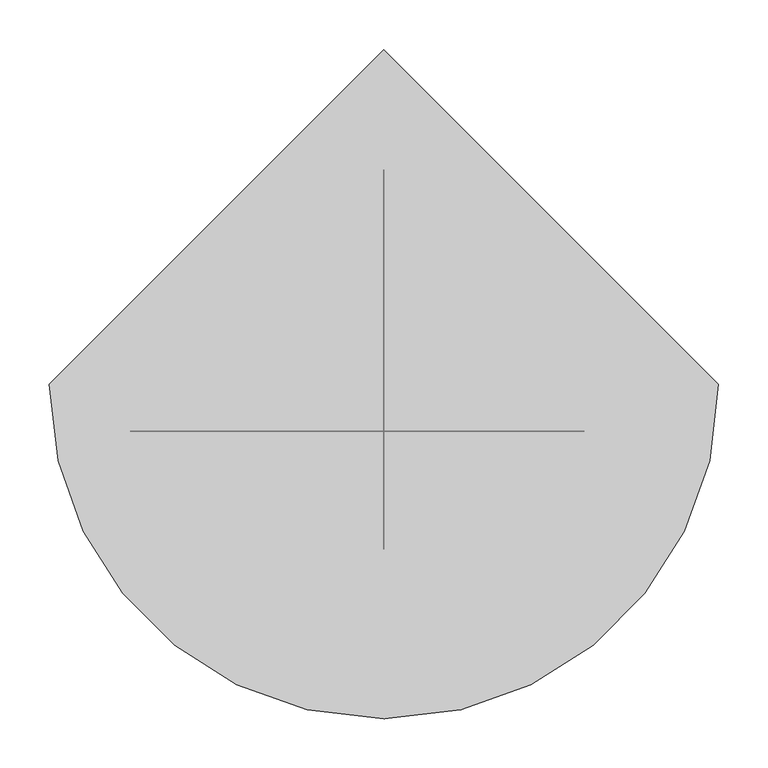
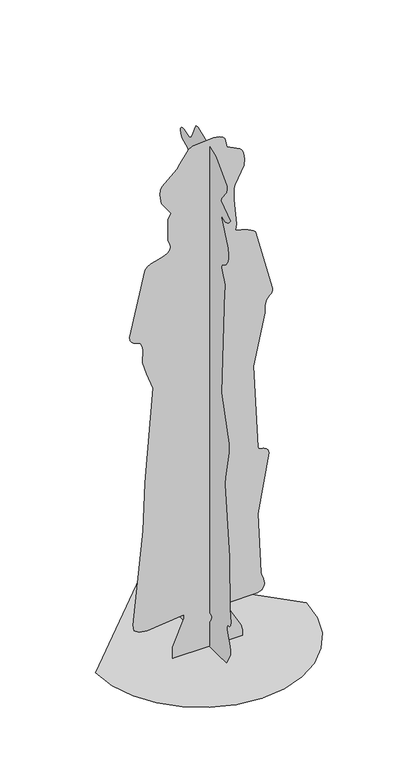
"""IFC4 building model written with IfcOpenShell, lengths in millimetres: proxy geometry, tina 23824 : tina 23824."""

import ifcopenshell
import ifcopenshell.guid

model = None  # the IFC model being written
_history = None  # IfcOwnerHistory: only IFC2X3 demands one
_inside = {}  # id of a spatial element -> (the spatial element, [elements in it])
_under = {}  # id of a project, library or spatial element -> (it, [spatial elements below it])
_declared = {}  # id of a project -> (the project, [libraries it declares])
_typed = {}  # id of a type object -> (the type object, [elements of that type])
_made_of = {}  # id of a material, layer set ... -> (it, [elements and type objects made of it])


def new_model(schema):
    """Start an empty IFC model of exactly this schema.

    Asked for "IFC4X3", IfcOpenShell would pick the latest addendum, in which some entities
    have other attributes; the version numbers below select the first issue.
    IFC2X3 requires an IfcOwnerHistory on every rooted entity: one is made here for all.
    """
    global model, _history
    if schema == "IFC4X3":
        model = ifcopenshell.file(schema_version=(4, 3, 0, 0))
    else:
        model = ifcopenshell.file(schema=schema)
    _inside.clear()
    _under.clear()
    _declared.clear()
    _typed.clear()
    _made_of.clear()
    _history = None
    if model.schema == "IFC2X3":
        org = make("IfcOrganization", Name="unknown")
        user = make(
            "IfcPersonAndOrganization",
            ThePerson=make("IfcPerson", FamilyName="unknown"),
            TheOrganization=org,
        )
        app = make(
            "IfcApplication",
            ApplicationDeveloper=org,
            Version="unknown",
            ApplicationFullName="unknown",
            ApplicationIdentifier="unknown",
        )
        _history = make(
            "IfcOwnerHistory",
            OwningUser=user,
            OwningApplication=app,
            ChangeAction="ADDED",
            CreationDate=0,
        )
    return model


def make(cls, **values):
    """One entity of the class cls with the attributes given. An attribute that is None is left unset."""
    return model.create_entity(
        cls, **{name: value for name, value in values.items() if value is not None}
    )


def rooted(cls, **values):
    """An entity with a GlobalId (a new one), such as an element, a storey or a relation."""
    return make(cls, GlobalId=ifcopenshell.guid.new(), OwnerHistory=_history, **values)


def si_unit(unit_type, name, prefix=None):
    """IfcSIUnit, for example si_unit("LENGTHUNIT", "METRE", prefix="MILLI")."""
    return make("IfcSIUnit", UnitType=unit_type, Prefix=prefix, Name=name)


def assignment(units):
    """IfcUnitAssignment: the units of a project."""
    return None if units is None else make("IfcUnitAssignment", Units=units)


def point(xyz):
    """IfcCartesianPoint."""
    return None if xyz is None else make("IfcCartesianPoint", Coordinates=xyz)


def direction(xyz):
    """IfcDirection."""
    return None if xyz is None else make("IfcDirection", DirectionRatios=xyz)


def frame(location, z_axis=None, x_axis=None):
    """IfcAxis2Placement3D, a coordinate frame: its origin and axes. An axis left out is left unset."""
    return make(
        "IfcAxis2Placement3D",
        Location=point(location),
        Axis=direction(z_axis),
        RefDirection=direction(x_axis),
    )


def origin():
    """The frame at (0, 0, 0) with its axes left unset."""
    return frame((0.0, 0.0, 0.0))


def place(relative_to, where):
    """IfcLocalPlacement: puts the frame where relative to a parent placement (None: the world)."""
    return make(
        "IfcLocalPlacement", PlacementRelTo=relative_to, RelativePlacement=where
    )


def context(
    kind, dimensions, precision=None, world=None, true_north=None, identifier=None
):
    """IfcGeometricRepresentationContext, for example the 3D "Model" context."""
    return make(
        "IfcGeometricRepresentationContext",
        ContextIdentifier=identifier,
        ContextType=kind,
        CoordinateSpaceDimension=dimensions,
        Precision=precision,
        WorldCoordinateSystem=world,
        TrueNorth=true_north,
    )


def project(units=None, contexts=None):
    """IfcProject with its units and contexts."""
    return rooted(
        "IfcProject",
        Name="project",
        RepresentationContexts=contexts,
        UnitsInContext=assignment(units),
    )


def spatial(cls, under=None, at=None, **own):
    """A site, building, storey or space (cls), placed at a placement, below another one or the project."""
    s = rooted(cls, ObjectPlacement=at, **own)
    if under is not None:
        _under.setdefault(under.id(), (under, []))[1].append(s)
    return s


def point_list(points):
    """IfcCartesianPointList2D or 3D."""
    cls = (
        "IfcCartesianPointList2D" if len(points[0]) == 2 else "IfcCartesianPointList3D"
    )
    return make(cls, CoordList=points)


def triangles(points, corners, closed=None, point_numbers=None):
    """IfcTriangulatedFaceSet: each triangle names its three corners, points numbered from 1."""
    return make(
        "IfcTriangulatedFaceSet",
        Coordinates=point_list(points),
        Closed=closed,
        CoordIndex=corners,
        PnIndex=point_numbers,
    )


def shape(context_of_items, identifier, shape_type, items):
    """IfcShapeRepresentation: the items that make up one representation, for example the "Body"."""
    return make(
        "IfcShapeRepresentation",
        ContextOfItems=context_of_items,
        RepresentationIdentifier=identifier,
        RepresentationType=shape_type,
        Items=items,
    )


def source(mapping_origin, context_of_items, identifier, shape_type, items):
    """IfcRepresentationMap: a shape defined once, which mapped items show again and again."""
    return make(
        "IfcRepresentationMap",
        MappingOrigin=mapping_origin,
        MappedRepresentation=shape(context_of_items, identifier, shape_type, items),
    )


def transform(
    local_origin,
    x_axis=None,
    y_axis=None,
    z_axis=None,
    scale=None,
    scale2=None,
    scale3=None,
    uniform=True,
):
    """IfcCartesianTransformationOperator3D, or its non-uniform kind. x_axis, y_axis, z_axis: its Axis1, 2, 3."""
    if uniform:
        return make(
            "IfcCartesianTransformationOperator3D",
            Axis1=direction(x_axis),
            Axis2=direction(y_axis),
            LocalOrigin=point(local_origin),
            Scale=scale,
            Axis3=direction(z_axis),
        )
    return make(
        "IfcCartesianTransformationOperator3DnonUniform",
        Axis1=direction(x_axis),
        Axis2=direction(y_axis),
        LocalOrigin=point(local_origin),
        Scale=scale,
        Axis3=direction(z_axis),
        Scale2=scale2,
        Scale3=scale3,
    )


def mapped(mapping_source, mapping_target):
    """IfcMappedItem: shows the shape of a source again, moved by a transform."""
    return make(
        "IfcMappedItem", MappingSource=mapping_source, MappingTarget=mapping_target
    )


def made_of(thing, what):
    """Note that an element or type object is made of a material, layer set ...; save() writes the relation."""
    if what is not None:
        _made_of.setdefault(what.id(), (what, []))[1].append(thing)
    return thing


def element(
    cls,
    number,
    at=None,
    inside=None,
    cuts=None,
    type_object=None,
    material=None,
    context=None,
    identifier="Body",
    shape_type=None,
    held_by="IfcProductDefinitionShape",
    body=None,
    shapes=None,
    **own,
):
    """One element of the class cls, such as IfcWall. Its Tag is "e" and its number.

    at: its placement. inside: the storey or other place that contains it. cuts: it is an
    opening in that element (IfcRelVoidsElement). A single representation is given by context,
    identifier, shape_type and body (its items); several are given by shapes. held_by: the class
    of the entity that holds the representations. save() writes the other relations.
    """
    e = rooted(cls, Tag="e%d" % number, ObjectPlacement=at, **own)
    if body is not None:
        shapes = [shape(context, identifier, shape_type, body)]
    if shapes is not None:
        e.Representation = make(held_by, Representations=shapes)
    if inside is not None:
        _inside.setdefault(inside.id(), (inside, []))[1].append(e)
    if cuts is not None:
        rooted(
            "IfcRelVoidsElement", RelatingBuildingElement=cuts, RelatedOpeningElement=e
        )
    if type_object is not None:
        _typed.setdefault(type_object.id(), (type_object, []))[1].append(e)
    return made_of(e, material)


def aggregate(whole, parts):
    """IfcRelAggregates: a whole, such as a stair, and the parts it consists of."""
    return rooted("IfcRelAggregates", RelatingObject=whole, RelatedObjects=parts)


def save(model, path):
    """Write the relations noted so far, then the file.

    IfcRelAggregates (storeys below a building ...), IfcRelContainedInSpatialStructure (elements
    in a storey), IfcRelDefinesByType, IfcRelAssociatesMaterial and IfcRelDeclares: one each for
    every whole, place, type object, material and project.
    """
    for whole, parts in _under.values():
        aggregate(whole, parts)
    for where, things in _inside.values():
        rooted(
            "IfcRelContainedInSpatialStructure",
            RelatedElements=things,
            RelatingStructure=where,
        )
    for kind, things in _typed.values():
        rooted("IfcRelDefinesByType", RelatedObjects=things, RelatingType=kind)
    for what, things in _made_of.values():
        rooted("IfcRelAssociatesMaterial", RelatedObjects=things, RelatingMaterial=what)
    for by, libraries in _declared.values():
        rooted("IfcRelDeclares", RelatingContext=by, RelatedDefinitions=libraries)
    model.write(path)


def entourage_2895b76d(model_context):
    return source(origin(), model_context, "Body", "Tessellation", [
        triangles([(-118.6024808, -47.6347378, 38.0857045), (-82.4820657, -47.6347378, 123.5964438), (-82.4078333, -47.6347378, 135.8076171), (-201.8741786, -47.6347378, 123.6873721), (-226.8996859, -47.6347378, 127.3924875), (-242.8002052, -47.6347378, 138.1060324), (-245.9828961, -47.6347378, 157.9872498), (-214.4620912, -47.6347378, 467.6612801), (-208.2590723, -47.6347378, 628.7997002), (-182.2156765, -47.6347378, 942.5936279), (-202.381742, -47.6347378, 998.3094131), (-215.4855752, -47.6347378, 1039.6297834), (-215.821474, -47.6347378, 1048.3149364), (-215.4215529, -47.6347378, 1056.8906485), (-214.7395452, -47.6347378, 1065.4273367), (-214.2301286, -47.6347378, 1073.9983252), (-214.3442568, -47.6347378, 1082.6741764), (-215.5356812, -47.6347378, 1091.525453), (-218.2581349, -47.6347378, 1100.6244616), (-222.7723761, -47.6347378, 1107.0752306), (-229.4309994, -47.6347378, 1111.2517199), (-237.153911, -47.6347378, 1114.3369967), (-244.8601449, -47.6347378, 1117.5141283), (-251.4686441, -47.6347378, 1121.9680716), (-255.900314, -47.6347378, 1128.8818211), (-257.0722446, -47.6347378, 1139.4385895), (-207.1678598, -47.6347378, 1352.9180008), (-199.4588645, -47.6347378, 1360.8821949), (-187.4852313, -47.6347378, 1366.7168678), (-173.049866, -47.6347378, 1371.2959488), (-157.9566194, -47.6347378, 1375.4901695), (-144.0093421, -47.6347378, 1380.175058), (-133.0118575, -47.6347378, 1386.2222179), (-126.7670806, -47.6347378, 1394.5047066), (-125.4318332, -47.6347378, 1401.2801651), (-127.4128987, -47.6347378, 1413.4282608), (-129.6649143, -47.6347378, 1418.6895676), (-132.0486895, -47.6347378, 1423.3336155), (-134.0325437, -47.6347378, 1427.3050301), (-132.6945168, -47.6347378, 1497.2715443), (-129.1053917, -47.6347378, 1508.7544189), (-123.9945118, -47.6347378, 1516.4930454), (-154.1540899, -47.6347378, 1559.4808285), (-159.7585988, -47.6347378, 1590.521957), (-157.2634749, -47.6347378, 1607.9849899), (-153.0368979, -47.6347378, 1617.2900906), (-104.5874569, -47.6347378, 1660.6611351), (-95.4448464, -47.6347378, 1675.8824444), (-68.2647649, -47.6347378, 1712.8963188), (-54.7860727, -47.6347378, 1720.8057198), (13.793251, -47.6347378, 1725.7013512), (32.0821851, -47.6347378, 1722.1345631), (43.5352696, -47.6347378, 1716.6933254), (49.9127328, -47.6347378, 1709.5716671), (56.2159682, -47.6347378, 1680.0680901), (98.2526783, -47.6347378, 1658.6643093), (104.3554853, -47.6347378, 1651.6019497), (108.8919907, -47.6347378, 1641.2540348), (113.2271458, -47.6347378, 1617.3336926), (111.7879713, -47.6347378, 1597.1945148), (82.8123962, -47.6347378, 1541.3868748), (78.3955873, -47.6347378, 1530.355862), (78.221143, -47.6347378, 1494.4090736), (81.1505245, -47.6347378, 1473.5952278), (87.0705392, -47.6347378, 1407.3950535), (83.9407248, -47.6347378, 1386.1879177), (93.3691283, -47.6347378, 1383.7559441), (103.6669826, -47.6347378, 1380.9944847), (114.2487677, -47.6347378, 1377.7940987), (124.5280548, -47.6347378, 1374.0491238), (133.9211951, -47.6347378, 1369.6499737), (141.84176, -47.6347378, 1364.4908409), (147.707027, -47.6347378, 1358.4631565), (203.1565494, -47.6347378, 1147.7562504), (202.6489859, -47.6347378, 1140.2068565), (200.5667729, -47.6347378, 1134.3935486), (197.3998514, -47.6347378, 1129.8329258), (193.6427769, -47.6347378, 1126.0442762), (189.7864171, -47.6347378, 1122.5442719), (186.3244191, -47.6347378, 1118.8530727), (183.7485589, -47.6347378, 1114.4863335), (180.7412388, -47.6347378, 1104.3026527), (179.3224846, -47.6347378, 1093.7014103), (178.983788, -47.6347378, 1082.7502619), (179.2129891, -47.6347378, 1071.5217321), (142.1618895, -47.6347378, 903.7795), (156.0237977, -47.6347378, 623.7611996), (158.5087296, -47.6347378, 617.7901251), (163.2567864, -47.6347378, 614.8626148), (169.444036, -47.6347378, 613.3956259), (176.2446201, -47.6347378, 611.8079321), (182.8317907, -47.6347378, 608.5166722), (188.3815792, -47.6347378, 601.9378587), (192.0662743, -47.6347378, 590.4912827), (156.0237977, -47.6347378, 396.418899), (165.8020344, -47.6347378, 192.9106632), (168.1922955, -47.6347378, 185.5199261), (170.9797162, -47.6347378, 177.5863805), (173.6307353, -47.6347378, 169.2955712), (175.6127183, -47.6347378, 160.8312623), (176.3903053, -47.6347378, 152.379934), (175.4317882, -47.6347378, 144.1253234), (168.3491173, -47.6347378, 133.8915095), (154.6421597, -47.6347378, 127.7701444), (58.9885369, -47.6347378, 127.4899107), (56.2159682, -47.6347378, 116.4005713), (101.0707112, -47.6347378, 37.0993457), (106.6641016, -47.6347378, 18.0541737), (105.8020812, -47.6347378, 0.0), (-118.3148258, -47.6347378, 0.0), (0.0, -54.5513123, 115.1627471), (0.0, -59.6705447, 112.2277973), (0.0, -61.6061461, 107.3080667), (0.0, -59.5796073, 99.6946324), (0.0, -52.8142817, 88.6758101), (0.0, -44.5346181, 79.7484662), (0.0, -38.0847779, 77.4212917), (0.0, -33.3088703, 80.3915047), (0.0, -30.0537933, 87.3554056), (0.0, -27.8620893, 119.17314), (0.0, -145.2091144, 6.8673968), (0.0, -161.5494597, 35.0431167), (0.0, -163.7123909, 41.543994), (0.0, -165.0513535, 56.4646448), (0.0, -162.6425252, 70.0333433), (0.0, -147.9891046, 107.0380432), (0.0, -145.6442986, 119.6101773), (0.0, -147.0779048, 133.0350483), (0.0, -159.447753, 133.9267635), (0.0, -165.7983101, 141.1708889), (0.0, -167.6643299, 152.8364559), (0.0, -161.6821551, 195.066182), (0.0, -158.8307121, 370.4998052), (0.0, -134.8528152, 604.4088561), (0.0, -137.4657826, 630.1117567), (0.0, -156.469192, 724.2417669), (0.0, -156.1305136, 755.5583874), (0.0, -114.2079362, 903.3962385), (0.0, -130.4434278, 1258.6544231), (0.0, -135.0133342, 1270.3422272), (0.0, -134.2635979, 1282.5153214), (0.0, -115.83826, 1329.7483395), (0.0, -116.8218301, 1339.6090748), (0.0, -129.4932496, 1346.1220493), (0.0, -140.4582598, 1355.1042046), (0.0, -148.9049463, 1366.6277744), (0.0, -154.0176883, 1380.767173), (0.0, -154.9836359, 1397.5927448), (0.0, -150.9899389, 1417.1778866), (0.0, -111.0354464, 1505.4037514), (0.0, -130.1557727, 1498.7358444), (0.0, -138.0614948, 1498.201284), (0.0, -145.1534401, 1499.6340454), (0.0, -151.6478203, 1503.109996), (0.0, -157.7617548, 1508.7042767), (0.0, -163.7123909, 1516.4930454), (0.0, -111.0354464, 1555.307246), (0.0, -115.3928657, 1565.6672241), (0.0, -142.5367576, 1601.7699623), (0.0, -145.4540849, 1612.318301), (0.0, -144.305336, 1624.6185677), (0.0, -83.3116117, 1688.3858963), (0.0, 16.4971557, 1727.1999516), (0.0, 26.1092848, 1726.2803856), (0.0, 33.1455581, 1716.0308659), (0.0, 45.9051286, 1684.0145061), (0.0, 54.8352521, 1670.4856808), (0.0, 67.6013152, 1664.1007507), (0.0, 95.5905225, 1672.8907665), (0.0, 103.6679091, 1673.2759174), (0.0, 109.6602941, 1670.5970112), (0.0, 113.1909561, 1665.3155022), (0.0, 113.8794588, 1657.8950249), (0.0, 111.3472188, 1648.7960163), (0.0, 105.2165701, 1638.4815296), (0.0, 102.2760519, 1635.7719566), (0.0, 74.7192446, 1624.6185677), (0.0, 65.7640681, 1614.5842964), (0.0, 62.4319768, 1602.0937798), (0.0, 63.3793663, 1588.1734085), (0.0, 83.0360199, 1538.6726509), (0.0, 77.4992394, 1529.7277027), (0.0, 75.4829062, 1476.4142418), (0.0, 71.8251217, 1469.4614685), (0.0, 16.4971557, 1466.5886787), (0.0, 16.4971557, 1366.7799454), (0.0, 18.8484578, 1360.1880512), (0.0, 52.539621, 1327.9657448), (0.0, 105.3622552, 1231.39911), (0.0, 120.552925, 982.93041), (0.0, 166.2103126, 823.3777943), (0.0, 167.4165798, 801.2900436), (0.0, 164.7089689, 783.190349), (0.0, 144.2060507, 730.9643944), (0.0, 144.0306798, 718.0239052), (0.0, 171.7554501, 645.9398603), (0.0, 186.7994991, 525.8657578), (0.0, 217.1038267, 449.5254684), (0.0, 217.3831338, 436.7788628), (0.0, 207.796982, 424.1436602), (0.0, 134.1002812, 404.8247449), (0.0, 105.2156435, 404.7365962), (0.0, 152.8058437, 209.5887513), (0.0, 152.0635198, 186.4487575), (0.0, 141.0131496, 169.2779487), (0.0, 115.8067122, 150.5668179), (0.0, 57.3786288, 128.2990456), (0.0, 49.7670522, 127.4899107), (0.0, 46.9944834, 116.4005713), (0.0, 56.6344519, 98.9615921), (0.0, 86.162119, 72.0468878), (0.0, 157.830428, 32.1499203), (0.0, 159.4356897, 29.2929136), (0.0, 159.4867404, 24.5244297), (0.0, 158.6367741, 18.6443187), (0.0, 157.534425, 12.4515065), (0.0, 156.8329416, 6.7467698), (0.0, 157.1827568, 2.3299599), (0.0, 159.2361925, 0.0), (0.0, -142.9329725, 0.0), (-339.3492356, 0.0, 0.0), (-330.3783079, -77.756264, 0.0), (-304.8276146, -149.1629065, 0.0), (-264.7450685, -212.1748216, 0.0), (-212.1748216, -264.7450685, 0.0), (-149.1629065, -304.8276146, 0.0), (-77.756264, -330.3783079, 0.0), (0.0, -339.3492356, 0.0), (77.756264, -330.3783079, 0.0), (149.1629065, -304.8276146, 0.0), (212.1748216, -264.7450685, 0.0), (264.7450685, -212.1748216, 0.0), (304.8276146, -149.1629065, 0.0), (330.3783079, -77.756264, 0.0), (339.3492356, 0.0, 0.0), (0.0, 339.3492356, 0.0)], [[108, 109, 110], [107, 108, 110], [107, 110, 1], [106, 107, 1], [106, 1, 2], [106, 2, 3], [105, 106, 3], [5, 6, 7], [4, 5, 7], [4, 7, 8], [3, 4, 8], [105, 3, 8], [104, 105, 8], [103, 104, 8], [102, 103, 8], [101, 102, 8], [100, 101, 8], [99, 100, 8], [98, 99, 8], [97, 98, 8], [96, 97, 8], [95, 96, 8], [95, 8, 9], [94, 95, 9], [93, 94, 9], [92, 93, 9], [91, 92, 9], [90, 91, 9], [89, 90, 9], [88, 89, 9], [87, 88, 9], [86, 87, 9], [86, 9, 10], [86, 10, 11], [85, 86, 11], [84, 85, 11], [84, 11, 12], [84, 12, 13], [84, 13, 14], [84, 14, 15], [84, 15, 16], [84, 16, 17], [83, 84, 17], [83, 17, 18], [82, 83, 18], [82, 18, 19], [81, 82, 19], [80, 81, 19], [80, 19, 20], [79, 80, 20], [78, 79, 20], [77, 78, 20], [76, 77, 20], [75, 76, 20], [74, 75, 20], [73, 74, 20], [72, 73, 20], [71, 72, 20], [70, 71, 20], [69, 70, 20], [68, 69, 20], [67, 68, 20], [66, 67, 20], [66, 20, 21], [66, 21, 22], [66, 22, 23], [66, 23, 24], [66, 24, 25], [66, 25, 26], [66, 26, 27], [66, 27, 28], [66, 28, 29], [66, 29, 30], [66, 30, 31], [66, 31, 32], [66, 32, 33], [66, 33, 34], [66, 34, 35], [65, 66, 35], [64, 65, 35], [64, 35, 36], [64, 36, 37], [63, 64, 37], [63, 37, 38], [63, 38, 39], [63, 39, 40], [63, 40, 41], [63, 41, 42], [62, 63, 42], [61, 62, 42], [61, 42, 43], [61, 43, 44], [61, 44, 45], [61, 45, 46], [61, 46, 47], [61, 47, 48], [60, 61, 48], [59, 60, 48], [58, 59, 48], [57, 58, 48], [56, 57, 48], [55, 56, 48], [55, 48, 49], [55, 49, 50], [55, 50, 51], [55, 51, 52], [55, 52, 53], [55, 53, 54], [218, 219, 220], [115, 123, 124], [115, 124, 125], [114, 115, 125], [114, 125, 126], [113, 114, 126], [113, 126, 127], [217, 218, 220], [155, 156, 157], [122, 123, 115], [122, 115, 116], [121, 122, 116], [216, 217, 220], [215, 216, 220], [214, 215, 220], [213, 214, 220], [212, 213, 220], [211, 212, 220], [210, 211, 220], [210, 220, 121], [209, 210, 121], [112, 113, 127], [112, 127, 128], [183, 184, 185], [180, 181, 182], [121, 116, 117], [209, 121, 117], [209, 117, 118], [209, 118, 119], [209, 119, 120], [208, 209, 120], [154, 155, 157], [153, 154, 157], [152, 153, 157], [151, 152, 157], [150, 151, 157], [163, 164, 165], [162, 163, 165], [162, 165, 166], [128, 129, 130], [128, 130, 131], [112, 128, 131], [112, 131, 132], [111, 112, 132], [120, 111, 132], [208, 120, 132], [208, 132, 133], [207, 208, 133], [206, 207, 133], [205, 206, 133], [204, 205, 133], [203, 204, 133], [202, 203, 133], [202, 133, 134], [182, 183, 185], [202, 134, 135], [180, 182, 185], [162, 166, 167], [161, 162, 167], [160, 161, 167], [159, 160, 167], [158, 159, 167], [157, 158, 167], [157, 167, 168], [150, 157, 168], [201, 202, 135], [200, 201, 135], [199, 200, 135], [198, 199, 135], [197, 198, 135], [196, 197, 135], [195, 196, 135], [195, 135, 136], [194, 195, 136], [194, 136, 137], [193, 194, 137], [192, 193, 137], [191, 192, 137], [191, 137, 138], [190, 191, 138], [190, 138, 139], [189, 190, 139], [188, 189, 139], [188, 139, 140], [188, 140, 141], [188, 141, 142], [187, 188, 142], [187, 142, 143], [186, 187, 143], [185, 186, 143], [185, 143, 144], [185, 144, 145], [185, 145, 146], [185, 146, 147], [185, 147, 148], [185, 148, 149], [185, 149, 150], [185, 150, 168], [170, 171, 172], [170, 172, 173], [169, 170, 173], [169, 173, 174], [169, 174, 175], [169, 175, 176], [168, 169, 176], [168, 176, 177], [168, 177, 178], [185, 168, 178], [185, 178, 179], [180, 185, 179], [235, 236, 221], [234, 235, 221], [234, 221, 222], [233, 234, 222], [233, 222, 223], [233, 223, 224], [232, 233, 224], [231, 232, 224], [231, 224, 225], [231, 225, 226], [231, 226, 227], [231, 227, 228], [231, 228, 229], [231, 229, 230]], closed=False),
    ])


if __name__ == "__main__":
    model = new_model("IFC4")
    model_context = context("Model", 3, world=origin())
    ifc_project = project(units=[si_unit("LENGTHUNIT", "METRE", prefix="MILLI")], contexts=[model_context])
    site = spatial("IfcSite", under=ifc_project)
    building = spatial("IfcBuilding", under=site)
    placement = place(None, origin())
    entourage_shape = entourage_2895b76d(model_context)
    element("IfcBuildingElementProxy", 1, Name="tina 23824 : tina 23824", ObjectType="tina 23824 : tina 23824", at=placement, inside=building, context=model_context, shape_type="MappedRepresentation", body=[
        mapped(entourage_shape, transform((0.0, 0.0, 0.0), x_axis=(1.0, 0.0, 0.0), y_axis=(0.0, 1.0, 0.0), z_axis=(0.0, 0.0, 1.0))),
    ])
    save(model, "model.ifc")

# Revit data of these elements
# Type "tina 23824 : tina 23824"
#   built-in parameter 1005195 = "RPC-8-E23G-6DS7-USQ4-G"
#   Height = 0
